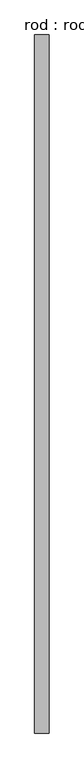
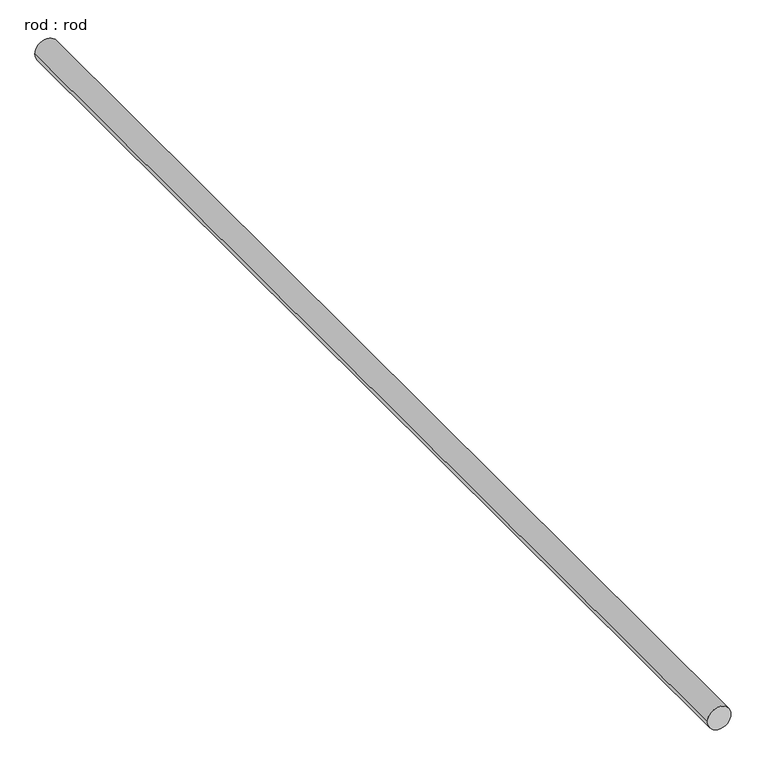
"""IFC4 building model written with IfcOpenShell, lengths in millimetres: proxy geometry, rod : rod."""

from ifc_helpers import new_model, si_unit, point, frame, frame_2d, origin, place, context, project, spatial, circle_curve, trimmed, segment, composite_curve, outline, extrude, source, transform, mapped, element, save


def rod_rod_da180fda(model_context):
    return source(origin(), model_context, "Body", "SweptSolid", [
        extrude(outline(composite_curve([segment(trimmed(circle_curve(frame_2d((0.0108462, 0.0)), 200.0), [point((0.0108462, 200.0))], [point((0.0108462, -200.0))], False, "CARTESIAN"), True, "CONTINUOUS"), segment(trimmed(circle_curve(frame_2d((0.0108462, 0.0)), 200.0), [point((0.0108462, -200.0))], [point((0.0108462, 200.0))], False, "CARTESIAN"), True, "CONTINUOUS")], self_intersect=False)), frame((0.0, -5741.610468, 0.0), z_axis=(0.0, 1.0, 0.0), x_axis=(0.0, 0.0, 1.0)), (0.0, 0.0, 1.0), 19668.6781667),
    ])


if __name__ == "__main__":
    model = new_model("IFC4")
    model_context = context("Model", 3, world=origin())
    ifc_project = project(units=[si_unit("LENGTHUNIT", "METRE", prefix="MILLI")], contexts=[model_context])
    site = spatial("IfcSite", under=ifc_project)
    building = spatial("IfcBuilding", under=site)
    placement = place(None, origin())
    rod_rod_shape = rod_rod_da180fda(model_context)
    element("IfcBuildingElementProxy", 1, Name="rod : rod", ObjectType="rod : rod", at=placement, inside=building, context=model_context, shape_type="MappedRepresentation", body=[
        mapped(rod_rod_shape, transform((0.0, 0.0, 0.0), x_axis=(1.0, 0.0, 0.0), y_axis=(0.0, 1.0, 0.0), z_axis=(0.0, 0.0, 1.0))),
    ])
    save(model, "model.ifc")

# Revit data of these elements
# Type "rod : rod"
#   Default Elevation = 0
